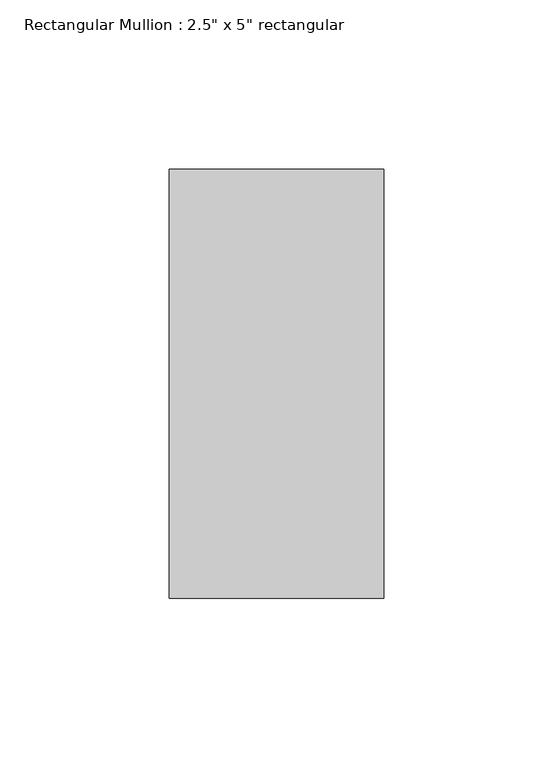
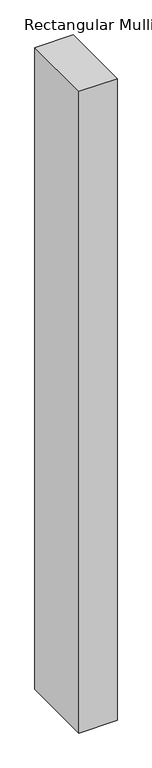
"""IFC4 building model written with IfcOpenShell, lengths in millimetres: member geometry."""

from ifc_helpers import new_model, si_unit, frame, origin, place, context, project, spatial, polyline, outline, extrude, source, transform, mapped, element, save


def member_4904f910(model_context):
    return source(origin(), model_context, "Body", "SweptSolid", [
        extrude(outline(polyline([(31.75, 63.5), (31.75, -63.5), (-31.75, -63.5), (-31.75, 63.5), (31.75, 63.5)])), frame((0.0, 0.0, -1130.3), z_axis=(0.0, 0.0, 1.0), x_axis=(1.0, 0.0, 0.0)), (0.0, 0.0, 1.0), 1130.3),
    ])


if __name__ == "__main__":
    model = new_model("IFC4")
    model_context = context("Model", 3, world=origin())
    ifc_project = project(units=[si_unit("LENGTHUNIT", "METRE", prefix="MILLI")], contexts=[model_context])
    site = spatial("IfcSite", under=ifc_project)
    building = spatial("IfcBuilding", under=site)
    placement = place(None, origin())
    member_shape = member_4904f910(model_context)
    element("IfcMember", 1, ObjectType="Rectangular Mullion : 2.5\" x 5\" rectangular", at=placement, inside=building, context=model_context, shape_type="MappedRepresentation", body=[
        mapped(member_shape, transform((0.0, 0.0, 0.0), x_axis=(1.0, 0.0, 0.0), y_axis=(0.0, 1.0, 0.0), z_axis=(0.0, 0.0, 1.0))),
    ])
    save(model, "model.ifc")

# Revit data of these elements
# Type "Rectangular Mullion : 2.5\" x 5\" rectangular"
#   built-in parameter 1007304 = 0.416667 (stored number, unit not read)
#   built-in parameter 1007301 = 0.104167 (stored number, unit not read)
#   built-in parameter 1007300 = 0.104167 (stored number, unit not read)
# Element 1 (IfcMember, "Rectangular Mullion : 2.5\" x 5\" rectangular")
#   Materials on its faces: "Metal - Aluminum"
# Materials
#   "Metal - Aluminum": class "Metal", colour RGB 140 140 140, transparency 0
